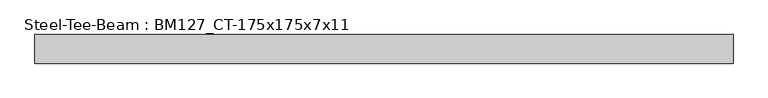
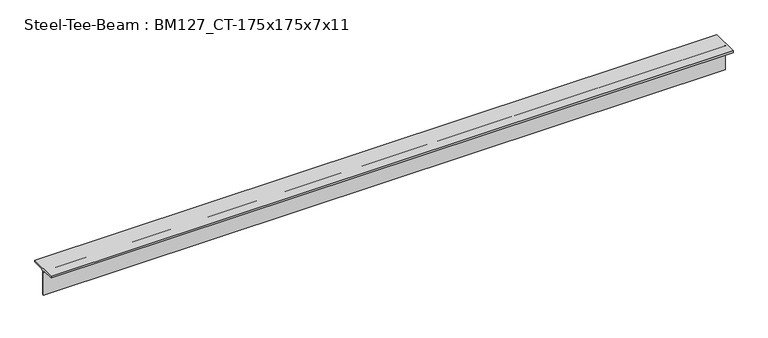
"""IFC4 building model written with IfcOpenShell, lengths in millimetres: beam geometry, Steel-Tee-Beam : BM127_CT-175x175x7x11."""

from ifc_helpers import new_model, si_unit, point, frame, frame_2d, origin, place, context, project, spatial, polyline, circle_curve, trimmed, segment, composite_curve, outline, extrude, source, transform, mapped, element, save


def steel_tee_beam_bm127_ct_175x175x7x11_58f75cbf(model_context):
    return source(origin(), model_context, "Body", "SweptSolid", [
        extrude(outline(composite_curve([segment(polyline([(-87.5, 87.5), (87.5, 87.5), (87.5, 76.5), (17.5, 76.5)]), True, "CONTINUOUS"), segment(trimmed(circle_curve(frame_2d((17.5, 62.5)), 14.0), [point((17.5, 76.5))], [point((3.5, 62.5))], True, "CARTESIAN"), True, "CONTINUOUS"), segment(polyline([(3.5, 62.5), (3.5, -87.5), (-3.5, -87.5), (-3.5, 62.5)]), True, "CONTINUOUS"), segment(trimmed(circle_curve(frame_2d((-17.5, 62.5)), 14.0), [point((-3.5, 62.5))], [point((-17.5, 76.5))], True, "CARTESIAN"), True, "CONTINUOUS"), segment(polyline([(-17.5, 76.5), (-87.5, 76.5), (-87.5, 87.5)]), True, "CONTINUOUS")], self_intersect=False)), frame((-2077.083277, 0.0, 0.0), z_axis=(1.0, 0.0, 0.0), x_axis=(0.0, 1.0, 0.0)), (0.0, 0.0, 1.0), 4261.3199196),
    ])


if __name__ == "__main__":
    model = new_model("IFC4")
    model_context = context("Model", 3, world=origin())
    ifc_project = project(units=[si_unit("LENGTHUNIT", "METRE", prefix="MILLI")], contexts=[model_context])
    site = spatial("IfcSite", under=ifc_project)
    building = spatial("IfcBuilding", under=site)
    placement = place(None, origin())
    steel_tee_beam_bm127_ct_175x175x7x11_shape = steel_tee_beam_bm127_ct_175x175x7x11_58f75cbf(model_context)
    element("IfcBeam", 1, ObjectType="Steel-Tee-Beam : BM127_CT-175x175x7x11", at=placement, inside=building, context=model_context, shape_type="MappedRepresentation", body=[
        mapped(steel_tee_beam_bm127_ct_175x175x7x11_shape, transform((0.0, 0.0, 0.0), x_axis=(1.0, 0.0, 0.0), y_axis=(0.0, 1.0, 0.0), z_axis=(0.0, 0.0, 1.0))),
    ])
    save(model, "model.ifc")

# Revit data of these elements
# Type "Steel-Tee-Beam : BM127_CT-175x175x7x11"
#   Section Area = 31.57 cm²
#   Mass per Unit Length = 24.80 kg/m
#   Length [instance default] = 1524 mm
#   bf = 175 mm
#   d = 175 mm
#   k = 25 mm
#   kr = 14 mm
#   tf = 11 mm
#   tw = 7 mm
#   hec_material4 [instance default] = none
#   hec_material3 [instance default] = none
#   hec_material2 [instance default] = none
#   hec_material1 [instance default] = none
#   Structural Material [instance default] = Steel, 45-345
#   Assembly Code = ""
# Element 1 (IfcBeam, "Steel-Tee-Beam : BM127_CT-175x175x7x11")
#   hec_material3 = F01AC000-00002_Building/Shelter Fire Proofing Work_Intumescent Coating Type_1 hr. rating (UL 1709))
#   hec_material1 = S03AA029-00001_Main Steel Structure Erection Work_Shelter/Building_Light Steel
#   Structural Material = S01AA003-00001_Main Steel Structure Fabrication Work_Shelter/Building_Light Steel - Standard
#   Materials on its faces: "S01AA003-00001_Main Steel Structure Fabrication Work_Shelter/Building_Light Steel - Standard"
# Materials
#   "Steel, 45-345": class "Metal", colour RGB 189 187 185, transparency 0, Description = "Steel 345 MPa", Cost = 0
#   "S01AA003-00001_Main Steel Structure Fabrication Work_Shelter/Building_Light Steel - Standard": class "Metal", colour RGB 120 120 120, transparency 0, Comments = "(30KG/M>Weight)", Description = "Structural steel 50ksi", W00) Work Master Code = "S01AA003-00001", W01) Work Master_Lv1 = "Main Steel Structure Fabrication Work", W02) Work Master_Lv2 = "Shelter/Building", W03) Work Master_Spec.1 = "Light Steel - Standard (30KG/M>Weight)", Cost = 0
#   "F01AC000-00002_Building/Shelter Fire Proofing Work_Intumescent Coating Type_1 hr. rating (UL 1709))": class "Metal", colour RGB 255 128 128, transparency 0, Description = "Paint finished steel", W00) Work Master Code = "F01AC000-00002", W01) Work Master_Lv1 = "Building/Shelter Fire Proofing Work", W02) Work Master_Lv2 = "Intumescent Coating Type", W03) Work Master_Spec.1 = "1 hr. rating (UL 1709)", Cost = 0
#   "S03AA029-00001_Main Steel Structure Erection Work_Shelter/Building_Light Steel": class "Metal", colour RGB 120 120 120, transparency 0, Comments = "(30KG/M>Weight)", Description = "Structural steel 50ksi", W00) Work Master Code = "S03AA029-00001", W01) Work Master_Lv1 = "Main Steel Structure Erection Work", W02) Work Master_Lv2 = "Shelter/Building", W03) Work Master_Spec.1 = "Light Steel (30KG/M>Weight)", Cost = 0
